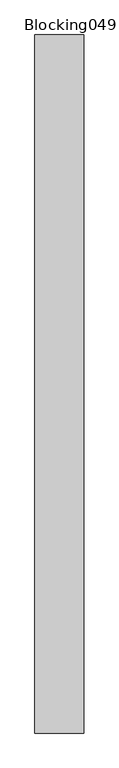
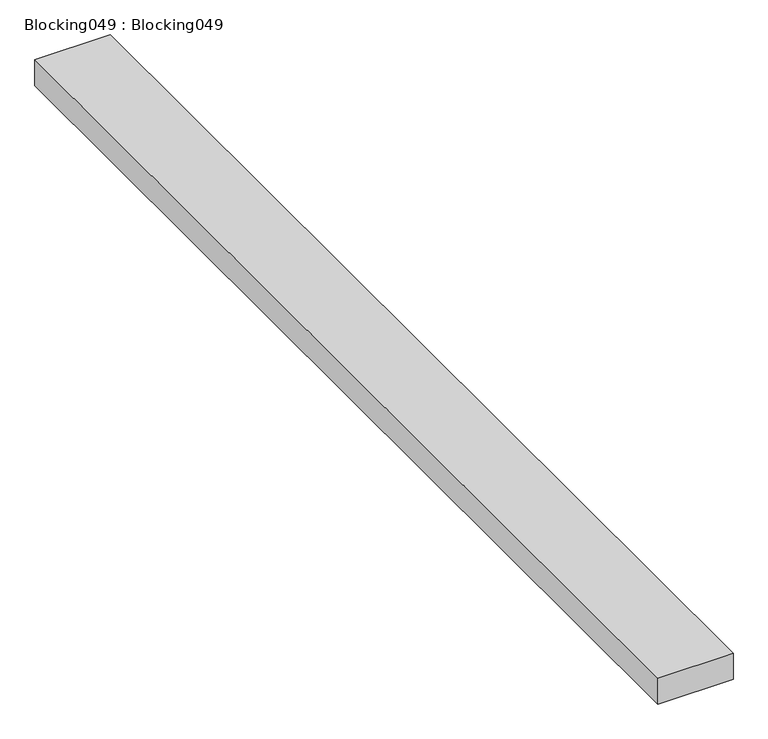
"""IFC4 building model written with IfcOpenShell, lengths in millimetres: proxy geometry, Blocking049 : Blocking049."""

from ifc_helpers import new_model, si_unit, frame, origin, place, context, project, spatial, polyline, outline, extrude, source, transform, mapped, element, save


def blocking049_blocking049_2d6d13d9(model_context):
    return source(origin(), model_context, "Body", "SweptSolid", [
        extrude(outline(polyline([(-950.3815411, -1052.8908936), (-1090.0815411, -1052.8908936), (-1090.0815411, 947.1091064), (-950.3815411, 947.1091064), (-950.3815411, -1052.8908936)])), frame((0.0, 0.0, 42083.0036692), z_axis=(0.0, 0.0, 1.0), x_axis=(1.0, 0.0, 0.0)), (0.0, 0.0, 1.0), 50.8),
    ])


if __name__ == "__main__":
    model = new_model("IFC4")
    model_context = context("Model", 3, world=origin())
    ifc_project = project(units=[si_unit("LENGTHUNIT", "METRE", prefix="MILLI")], contexts=[model_context])
    site = spatial("IfcSite", under=ifc_project)
    building = spatial("IfcBuilding", under=site)
    placement = place(None, origin())
    blocking049_blocking049_shape = blocking049_blocking049_2d6d13d9(model_context)
    element("IfcBuildingElementProxy", 1, Name="Blocking049 : Blocking049", ObjectType="Blocking049 : Blocking049", at=placement, inside=building, context=model_context, shape_type="MappedRepresentation", body=[
        mapped(blocking049_blocking049_shape, transform((0.0, 0.0, 0.0), x_axis=(1.0, 0.0, 0.0), y_axis=(0.0, 1.0, 0.0), z_axis=(0.0, 0.0, 1.0))),
    ])
    save(model, "model.ifc")

# Revit data of these elements
# Type "Blocking049 : Blocking049"
#   NameOverride = "Blocking049"
# Element 1 (IfcBuildingElementProxy, "Blocking049 : Blocking049")
#   Materials on its faces: "WOOD BLOCKING AS REQUIRED"
# Materials
#   "WOOD BLOCKING AS REQUIRED": class "Unassigned", colour RGB 166 124 85, transparency 0, Cost = 0
